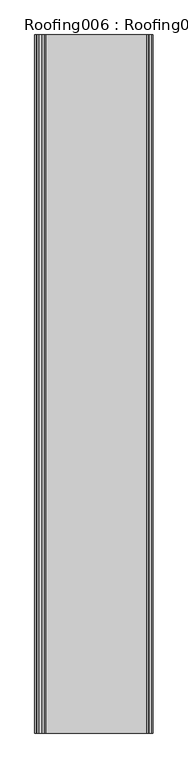
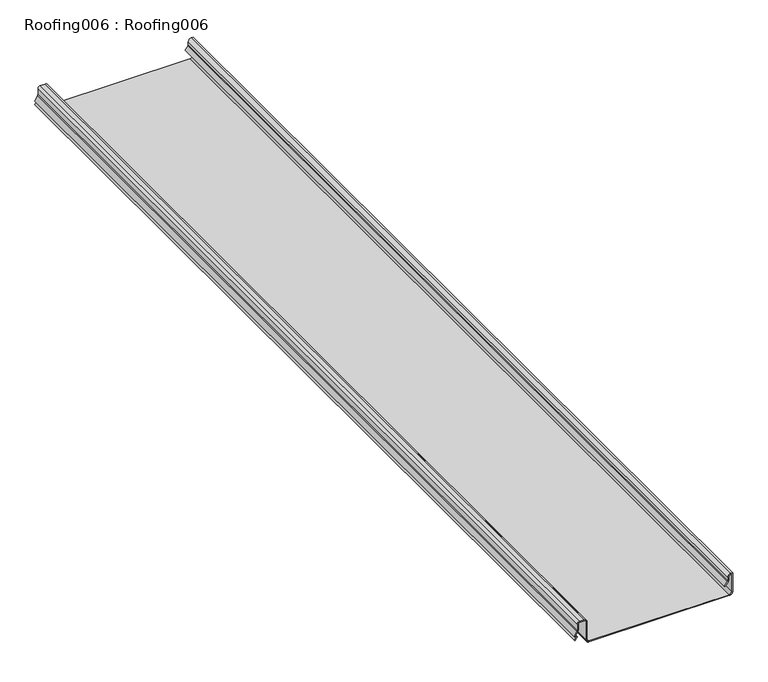
"""IFC4 building model written with IfcOpenShell, lengths in millimetres: proxy geometry, Roofing006 : Roofing006."""

from ifc_helpers import new_model, si_unit, point, frame, frame_2d, origin, place, context, project, spatial, polyline, circle_curve, trimmed, segment, composite_curve, outline, extrude, source, transform, mapped, element, save


def roofing006_roofing006_02cdabe2(model_context):
    return source(origin(), model_context, "Body", "SweptSolid", [
        extrude(outline(composite_curve([segment(trimmed(circle_curve(frame_2d((42571.8416239, -1174.390951)), 5.08), [point((42568.8585944, -1170.279025))], [point((42571.8416239, -1169.310951))], False, "CARTESIAN"), True, "CONTINUOUS"), segment(polyline([(42571.8416239, -1169.310951), (42578.5981823, -1169.310951)]), True, "CONTINUOUS"), segment(trimmed(circle_curve(frame_2d((42578.5981823, -1164.230951)), 5.08), [point((42578.5981823, -1169.310951))], [point((42583.6781823, -1164.230951))], True, "CARTESIAN"), True, "CONTINUOUS"), segment(polyline([(42583.6781823, -1164.230951), (42583.6781823, -1162.6361463), (42543.9409948, -1162.6361463)]), True, "CONTINUOUS"), segment(trimmed(circle_curve(frame_2d((42543.9409948, -1167.7161463)), 5.08), [point((42543.9409948, -1162.6361463))], [point((42538.8609948, -1167.7161463))], True, "CARTESIAN"), True, "CONTINUOUS"), segment(polyline([(42538.8609948, -1167.7161463), (42538.8609948, -1467.9902283)]), True, "CONTINUOUS"), segment(trimmed(circle_curve(frame_2d((42543.9409948, -1467.9902283)), 5.08), [point((42538.8609948, -1467.9902283))], [point((42543.9409948, -1473.0702283))], True, "CARTESIAN"), True, "CONTINUOUS"), segment(polyline([(42543.9409948, -1473.0702283), (42585.5544323, -1473.0702283)]), True, "CONTINUOUS"), segment(trimmed(circle_curve(frame_2d((42585.5544323, -1478.1502283)), 5.08), [point((42585.5544323, -1473.0702283))], [point((42590.6344323, -1478.1502283))], False, "CARTESIAN"), True, "CONTINUOUS"), segment(polyline([(42590.6344323, -1478.1502283), (42590.6344323, -1488.1580052)]), True, "CONTINUOUS"), segment(trimmed(circle_curve(frame_2d((42585.5544323, -1488.1580052)), 5.08), [point((42590.6344323, -1488.1580052))], [point((42585.5544323, -1493.2380052))], False, "CARTESIAN"), True, "CONTINUOUS"), segment(polyline([(42585.5544323, -1493.2380052), (42572.3718581, -1493.2380052)]), True, "CONTINUOUS"), segment(trimmed(circle_curve(frame_2d((42572.3718581, -1498.3180052)), 5.08), [point((42572.3718581, -1493.2380052))], [point((42569.8678467, -1493.8980135))], True, "CARTESIAN"), True, "CONTINUOUS"), segment(polyline([(42569.8678467, -1493.8980135), (42559.3102135, -1499.8791185), (42556.8688073, -1495.715056), (42551.2672448, -1499.7140794), (42550.1051711, -1498.0863249), (42557.4874863, -1492.8160005), (42560.0388845, -1497.1676653), (42568.8820154, -1492.1578593)]), True, "CONTINUOUS"), segment(trimmed(circle_curve(frame_2d((42572.3718581, -1498.3180052)), 7.08), [point((42568.8820154, -1492.1578593))], [point((42572.3718581, -1491.2380052))], False, "CARTESIAN"), True, "CONTINUOUS"), segment(polyline([(42572.3718581, -1491.2380052), (42585.5544323, -1491.2380052)]), True, "CONTINUOUS"), segment(trimmed(circle_curve(frame_2d((42585.5544323, -1488.1580052)), 3.08), [point((42585.5544323, -1491.2380052))], [point((42588.6344323, -1488.1580052))], True, "CARTESIAN"), True, "CONTINUOUS"), segment(polyline([(42588.6344323, -1488.1580052), (42588.6344323, -1478.1502283)]), True, "CONTINUOUS"), segment(trimmed(circle_curve(frame_2d((42585.5544323, -1478.1502283)), 3.08), [point((42588.6344323, -1478.1502283))], [point((42585.5544323, -1475.0702283))], True, "CARTESIAN"), True, "CONTINUOUS"), segment(polyline([(42585.5544323, -1475.0702283), (42543.9409948, -1475.0702283)]), True, "CONTINUOUS"), segment(trimmed(circle_curve(frame_2d((42543.9409948, -1467.9902283)), 7.08), [point((42543.9409948, -1475.0702283))], [point((42536.8609948, -1467.9902283))], False, "CARTESIAN"), True, "CONTINUOUS"), segment(polyline([(42536.8609948, -1467.9902283), (42536.8609948, -1167.7161463)]), True, "CONTINUOUS"), segment(trimmed(circle_curve(frame_2d((42543.9409948, -1167.7161463)), 7.08), [point((42536.8609948, -1167.7161463))], [point((42543.9409948, -1160.6361463))], False, "CARTESIAN"), True, "CONTINUOUS"), segment(polyline([(42543.9409948, -1160.6361463), (42585.6781823, -1160.6361463), (42585.6781823, -1164.230951)]), True, "CONTINUOUS"), segment(trimmed(circle_curve(frame_2d((42578.5981823, -1164.230951)), 7.08), [point((42585.6781823, -1164.230951))], [point((42578.5981823, -1171.310951))], False, "CARTESIAN"), True, "CONTINUOUS"), segment(polyline([(42578.5981823, -1171.310951), (42571.8416239, -1171.310951)]), True, "CONTINUOUS"), segment(trimmed(circle_curve(frame_2d((42571.8416239, -1174.390951)), 3.08), [point((42571.8416239, -1171.310951))], [point((42570.0330155, -1171.8978935))], True, "CARTESIAN"), True, "CONTINUOUS"), segment(polyline([(42570.0330155, -1171.8978935), (42561.5588533, -1178.0455421), (42560.3844323, -1176.4266736), (42568.8585944, -1170.279025)]), True, "CONTINUOUS")], self_intersect=False)), frame((0.0, -1052.8906574, 0.0), z_axis=(0.0, 1.0, 0.0), x_axis=(0.0, 0.0, 1.0)), (0.0, 0.0, 1.0), 2000.0),
    ])


if __name__ == "__main__":
    model = new_model("IFC4")
    model_context = context("Model", 3, world=origin())
    ifc_project = project(units=[si_unit("LENGTHUNIT", "METRE", prefix="MILLI")], contexts=[model_context])
    site = spatial("IfcSite", under=ifc_project)
    building = spatial("IfcBuilding", under=site)
    placement = place(None, origin())
    roofing006_roofing006_shape = roofing006_roofing006_02cdabe2(model_context)
    element("IfcBuildingElementProxy", 1, Name="Roofing006 : Roofing006", ObjectType="Roofing006 : Roofing006", at=placement, inside=building, context=model_context, shape_type="MappedRepresentation", body=[
        mapped(roofing006_roofing006_shape, transform((0.0, 0.0, 0.0), x_axis=(1.0, 0.0, 0.0), y_axis=(0.0, 1.0, 0.0), z_axis=(0.0, 0.0, 1.0))),
    ])
    save(model, "model.ifc")

# Revit data of these elements
# Type "Roofing006 : Roofing006"
#   NameOverride = "Roofing006"
# Element 1 (IfcBuildingElementProxy, "Roofing006 : Roofing006")
#   Materials on its faces: "STANDING SEAM METAL ROOF FOLLOW MANU. RECOMMENDED EDGE/TRANSITION DETAILS"
# Materials
#   "STANDING SEAM METAL ROOF FOLLOW MANU. RECOMMENDED EDGE/TRANSITION DETAILS": class "Unassigned", colour RGB 128 128 128, transparency 0, Cost = 0
